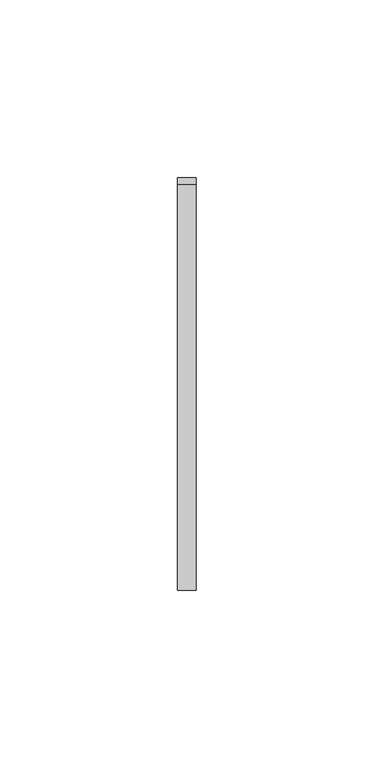
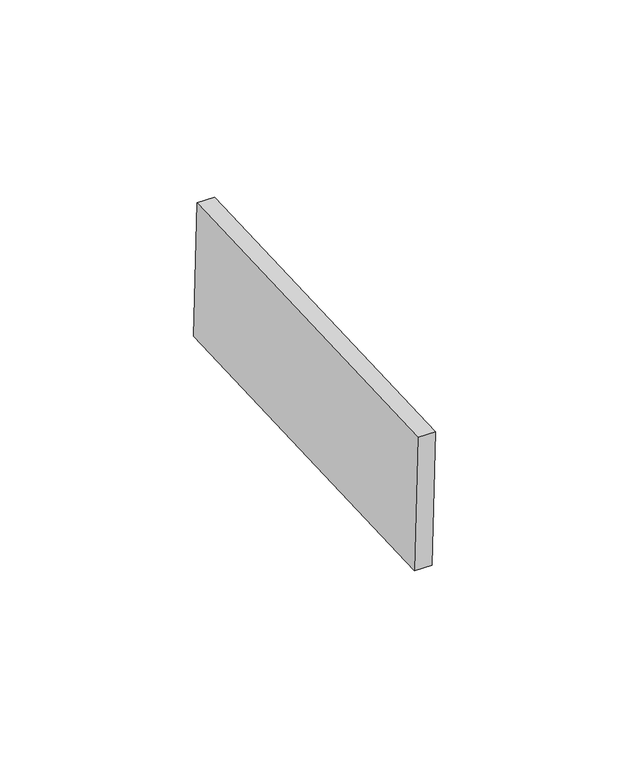
"""IFC4 building model written with IfcOpenShell, lengths in millimetres: proxy geometry, Inner panel:Inner panel:1:Inner panel:1 : Inner panel:Inner panel:300324:2:Inner panel:1:Inner panel:1 : Inner panel:Inner panel:300324:2 : Inner panel:Inner panel:1:Inner panel:1 : Inner panel:Inner panel:300324:300043:97 : Inner panel:Inner panel:1:Inner panel:1 : Inner panel:Inner panel:300324:2:Inner panel:1:Inner panel:1 : Inner panel:Inner panel:300324:2 : Inner panel:Inner panel:1:Inner panel:1 : Inner panel:Inner panel:300324:300043:308120."""

from ifc_helpers import new_model, si_unit, frame, origin, place, context, project, spatial, polyline, outline, extrude, source, transform, mapped, element, save


def generic_models_b743f119(model_context):
    return source(origin(), model_context, "Body", "SweptSolid", [
        extrude(outline(polyline([(0.0, -114.3), (0.0, 0.0), (5.2138089, 0.0), (5.2138089, -114.3), (0.0, -114.3)])), frame((593936.595117, -579007.2622385, 3952.103089), z_axis=(0.0, -0.04163054471216399, 0.9991330730923527), x_axis=(-1.0, 0.0, 0.0)), (0.0, 0.0, 1.0), 43.2233908),
    ])


if __name__ == "__main__":
    model = new_model("IFC4")
    model_context = context("Model", 3, world=origin())
    ifc_project = project(units=[si_unit("LENGTHUNIT", "METRE", prefix="MILLI")], contexts=[model_context])
    site = spatial("IfcSite", under=ifc_project)
    building = spatial("IfcBuilding", under=site)
    placement = place(None, origin())
    generic_models_shape = generic_models_b743f119(model_context)
    element("IfcBuildingElementProxy", 1, Name="Inner panel:Inner panel:1:Inner panel:1 : Inner panel:Inner panel:300324:2:Inner panel:1:Inner panel:1 : Inner panel:Inner panel:300324:2 : Inner panel:Inner panel:1:Inner panel:1 : Inner panel:Inner panel:300324:300043:97 : Inner panel:Inner panel:1:Inner panel:1 : Inner panel:Inner panel:300324:2:Inner panel:1:Inner panel:1 : Inner panel:Inner panel:300324:2 : Inner panel:Inner panel:1:Inner panel:1 : Inner panel:Inner panel:300324:300043:308120", ObjectType="Inner panel:Inner panel:1:Inner panel:1 : Inner panel:Inner panel:300324:2:Inner panel:1:Inner panel:1 : Inner panel:Inner panel:300324:2 : Inner panel:Inner panel:1:Inner panel:1 : Inner panel:Inner panel:300324:300043:97 : Inner panel:Inner panel:1:Inner panel:1 : Inner panel:Inner panel:300324:2:Inner panel:1:Inner panel:1 : Inner panel:Inner panel:300324:2 : Inner panel:Inner panel:1:Inner panel:1 : Inner panel:Inner panel:300324:300043:308120", at=placement, inside=building, context=model_context, shape_type="MappedRepresentation", body=[
        mapped(generic_models_shape, transform((0.0, 0.0, 0.0), x_axis=(1.0, 0.0, 0.0), y_axis=(0.0, 1.0, 0.0), z_axis=(0.0, 0.0, 1.0))),
    ])
    save(model, "model.ifc")

# Revit data of these elements
# Type "Inner panel:Inner panel:1:Inner panel:1 : Inner panel:Inner panel:300324:2:Inner panel:1:Inner panel:1 : Inner panel:Inner panel:300324:2 : Inner panel:Inner panel:1:Inner panel:1 : Inner panel:Inner panel:300324:300043:97 : Inner panel:Inner panel:1:Inner panel:1 : Inner panel:Inner panel:300324:2:Inner panel:1:Inner panel:1 : Inner panel:Inner panel:300324:2 : Inner panel:Inner panel:1:Inner panel:1 : Inner panel:Inner panel:300324:300043:308120"
#   NameOverride = "Inner panel:Inner panel:1:Inner panel:1 : Inner panel:Inner panel:300324:2:Inner panel:1:Inner panel:1 : Inner panel:Inner panel:300324:2 : Inner panel:Inner panel:1:Inner panel:1 : Inner panel:Inner panel:300324:300043:308120"
#   ObjectTypeOverride = "Inner panel:1:Inner panel:1 : Inner panel:Inner panel:300324:2 : Inner panel:Inner panel:1:Inner panel:1 : Inner panel:Inner panel:300324:300043"
#   Reference = "Inner panel"
#   Tag = "308120"
# Element 1 (IfcBuildingElementProxy, "Inner panel:Inner panel:1:Inner panel:1 : Inner panel:Inner panel:300324:2:Inner panel:1:Inner panel:1 : Inner panel:Inner panel:300324:2 : Inner panel:Inner panel:1:Inner panel:1 : Inner panel:Inner panel:300324:300043:97 : Inner panel:Inner panel:1:Inner panel:1 : Inner panel:Inner panel:300324:2:Inner panel:1:Inner panel:1 : Inner panel:Inner panel:300324:2 : Inner panel:Inner panel:1:Inner panel:1 : Inner panel:Inner panel:300324:300043:308120")
#   Materials on its faces: "SLIDING CLIP"
# Materials
#   "SLIDING CLIP": class "Generic", colour RGB 120 120 120, transparency 0, Cost = 0
